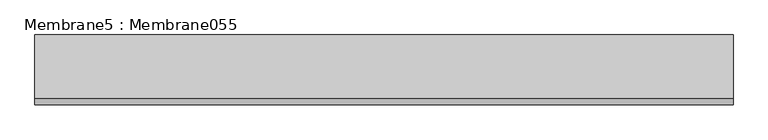
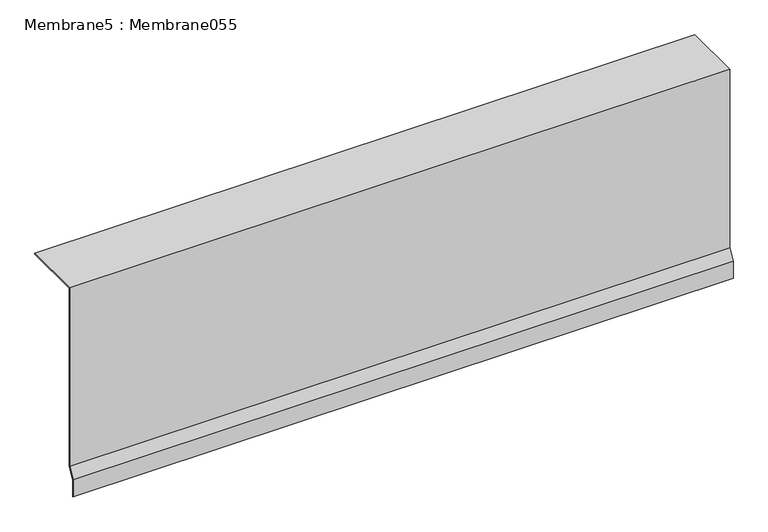
"""IFC4 building model written with IfcOpenShell, lengths in millimetres: proxy geometry, Membrane5 : Membrane055."""

import ifcopenshell
import ifcopenshell.guid

model = None  # the IFC model being written
_history = None  # IfcOwnerHistory: only IFC2X3 demands one
_inside = {}  # id of a spatial element -> (the spatial element, [elements in it])
_under = {}  # id of a project, library or spatial element -> (it, [spatial elements below it])
_declared = {}  # id of a project -> (the project, [libraries it declares])
_typed = {}  # id of a type object -> (the type object, [elements of that type])
_made_of = {}  # id of a material, layer set ... -> (it, [elements and type objects made of it])


def new_model(schema):
    """Start an empty IFC model of exactly this schema.

    Asked for "IFC4X3", IfcOpenShell would pick the latest addendum, in which some entities
    have other attributes; the version numbers below select the first issue.
    IFC2X3 requires an IfcOwnerHistory on every rooted entity: one is made here for all.
    """
    global model, _history
    if schema == "IFC4X3":
        model = ifcopenshell.file(schema_version=(4, 3, 0, 0))
    else:
        model = ifcopenshell.file(schema=schema)
    _inside.clear()
    _under.clear()
    _declared.clear()
    _typed.clear()
    _made_of.clear()
    _history = None
    if model.schema == "IFC2X3":
        org = make("IfcOrganization", Name="unknown")
        user = make(
            "IfcPersonAndOrganization",
            ThePerson=make("IfcPerson", FamilyName="unknown"),
            TheOrganization=org,
        )
        app = make(
            "IfcApplication",
            ApplicationDeveloper=org,
            Version="unknown",
            ApplicationFullName="unknown",
            ApplicationIdentifier="unknown",
        )
        _history = make(
            "IfcOwnerHistory",
            OwningUser=user,
            OwningApplication=app,
            ChangeAction="ADDED",
            CreationDate=0,
        )
    return model


def make(cls, **values):
    """One entity of the class cls with the attributes given. An attribute that is None is left unset."""
    return model.create_entity(
        cls, **{name: value for name, value in values.items() if value is not None}
    )


def rooted(cls, **values):
    """An entity with a GlobalId (a new one), such as an element, a storey or a relation."""
    return make(cls, GlobalId=ifcopenshell.guid.new(), OwnerHistory=_history, **values)


def si_unit(unit_type, name, prefix=None):
    """IfcSIUnit, for example si_unit("LENGTHUNIT", "METRE", prefix="MILLI")."""
    return make("IfcSIUnit", UnitType=unit_type, Prefix=prefix, Name=name)


def assignment(units):
    """IfcUnitAssignment: the units of a project."""
    return None if units is None else make("IfcUnitAssignment", Units=units)


def point(xyz):
    """IfcCartesianPoint."""
    return None if xyz is None else make("IfcCartesianPoint", Coordinates=xyz)


def direction(xyz):
    """IfcDirection."""
    return None if xyz is None else make("IfcDirection", DirectionRatios=xyz)


def frame(location, z_axis=None, x_axis=None):
    """IfcAxis2Placement3D, a coordinate frame: its origin and axes. An axis left out is left unset."""
    return make(
        "IfcAxis2Placement3D",
        Location=point(location),
        Axis=direction(z_axis),
        RefDirection=direction(x_axis),
    )


def origin():
    """The frame at (0, 0, 0) with its axes left unset."""
    return frame((0.0, 0.0, 0.0))


def place(relative_to, where):
    """IfcLocalPlacement: puts the frame where relative to a parent placement (None: the world)."""
    return make(
        "IfcLocalPlacement", PlacementRelTo=relative_to, RelativePlacement=where
    )


def context(
    kind, dimensions, precision=None, world=None, true_north=None, identifier=None
):
    """IfcGeometricRepresentationContext, for example the 3D "Model" context."""
    return make(
        "IfcGeometricRepresentationContext",
        ContextIdentifier=identifier,
        ContextType=kind,
        CoordinateSpaceDimension=dimensions,
        Precision=precision,
        WorldCoordinateSystem=world,
        TrueNorth=true_north,
    )


def project(units=None, contexts=None):
    """IfcProject with its units and contexts."""
    return rooted(
        "IfcProject",
        Name="project",
        RepresentationContexts=contexts,
        UnitsInContext=assignment(units),
    )


def spatial(cls, under=None, at=None, **own):
    """A site, building, storey or space (cls), placed at a placement, below another one or the project."""
    s = rooted(cls, ObjectPlacement=at, **own)
    if under is not None:
        _under.setdefault(under.id(), (under, []))[1].append(s)
    return s


def polyline(points):
    """IfcPolyline through the points."""
    return make("IfcPolyline", Points=[point(p) for p in points])


def outline(outer, holes=None, kind="AREA"):
    """IfcArbitraryClosedProfileDef: a profile drawn as a closed curve; with holes, ...WithVoids."""
    if holes is None:
        return make("IfcArbitraryClosedProfileDef", ProfileType=kind, OuterCurve=outer)
    return make(
        "IfcArbitraryProfileDefWithVoids",
        ProfileType=kind,
        OuterCurve=outer,
        InnerCurves=holes,
    )


def extrude(swept, where, along, depth):
    """IfcExtrudedAreaSolid: the profile swept, set in the frame where, extruded along a direction by depth."""
    return make(
        "IfcExtrudedAreaSolid",
        SweptArea=swept,
        Position=where,
        ExtrudedDirection=direction(along),
        Depth=depth,
    )


def shape(context_of_items, identifier, shape_type, items):
    """IfcShapeRepresentation: the items that make up one representation, for example the "Body"."""
    return make(
        "IfcShapeRepresentation",
        ContextOfItems=context_of_items,
        RepresentationIdentifier=identifier,
        RepresentationType=shape_type,
        Items=items,
    )


def source(mapping_origin, context_of_items, identifier, shape_type, items):
    """IfcRepresentationMap: a shape defined once, which mapped items show again and again."""
    return make(
        "IfcRepresentationMap",
        MappingOrigin=mapping_origin,
        MappedRepresentation=shape(context_of_items, identifier, shape_type, items),
    )


def transform(
    local_origin,
    x_axis=None,
    y_axis=None,
    z_axis=None,
    scale=None,
    scale2=None,
    scale3=None,
    uniform=True,
):
    """IfcCartesianTransformationOperator3D, or its non-uniform kind. x_axis, y_axis, z_axis: its Axis1, 2, 3."""
    if uniform:
        return make(
            "IfcCartesianTransformationOperator3D",
            Axis1=direction(x_axis),
            Axis2=direction(y_axis),
            LocalOrigin=point(local_origin),
            Scale=scale,
            Axis3=direction(z_axis),
        )
    return make(
        "IfcCartesianTransformationOperator3DnonUniform",
        Axis1=direction(x_axis),
        Axis2=direction(y_axis),
        LocalOrigin=point(local_origin),
        Scale=scale,
        Axis3=direction(z_axis),
        Scale2=scale2,
        Scale3=scale3,
    )


def mapped(mapping_source, mapping_target):
    """IfcMappedItem: shows the shape of a source again, moved by a transform."""
    return make(
        "IfcMappedItem", MappingSource=mapping_source, MappingTarget=mapping_target
    )


def made_of(thing, what):
    """Note that an element or type object is made of a material, layer set ...; save() writes the relation."""
    if what is not None:
        _made_of.setdefault(what.id(), (what, []))[1].append(thing)
    return thing


def element(
    cls,
    number,
    at=None,
    inside=None,
    cuts=None,
    type_object=None,
    material=None,
    context=None,
    identifier="Body",
    shape_type=None,
    held_by="IfcProductDefinitionShape",
    body=None,
    shapes=None,
    **own,
):
    """One element of the class cls, such as IfcWall. Its Tag is "e" and its number.

    at: its placement. inside: the storey or other place that contains it. cuts: it is an
    opening in that element (IfcRelVoidsElement). A single representation is given by context,
    identifier, shape_type and body (its items); several are given by shapes. held_by: the class
    of the entity that holds the representations. save() writes the other relations.
    """
    e = rooted(cls, Tag="e%d" % number, ObjectPlacement=at, **own)
    if body is not None:
        shapes = [shape(context, identifier, shape_type, body)]
    if shapes is not None:
        e.Representation = make(held_by, Representations=shapes)
    if inside is not None:
        _inside.setdefault(inside.id(), (inside, []))[1].append(e)
    if cuts is not None:
        rooted(
            "IfcRelVoidsElement", RelatingBuildingElement=cuts, RelatedOpeningElement=e
        )
    if type_object is not None:
        _typed.setdefault(type_object.id(), (type_object, []))[1].append(e)
    return made_of(e, material)


def aggregate(whole, parts):
    """IfcRelAggregates: a whole, such as a stair, and the parts it consists of."""
    return rooted("IfcRelAggregates", RelatingObject=whole, RelatedObjects=parts)


def save(model, path):
    """Write the relations noted so far, then the file.

    IfcRelAggregates (storeys below a building ...), IfcRelContainedInSpatialStructure (elements
    in a storey), IfcRelDefinesByType, IfcRelAssociatesMaterial and IfcRelDeclares: one each for
    every whole, place, type object, material and project.
    """
    for whole, parts in _under.values():
        aggregate(whole, parts)
    for where, things in _inside.values():
        rooted(
            "IfcRelContainedInSpatialStructure",
            RelatedElements=things,
            RelatingStructure=where,
        )
    for kind, things in _typed.values():
        rooted("IfcRelDefinesByType", RelatedObjects=things, RelatingType=kind)
    for what, things in _made_of.values():
        rooted("IfcRelAssociatesMaterial", RelatedObjects=things, RelatingMaterial=what)
    for by, libraries in _declared.values():
        rooted("IfcRelDeclares", RelatingContext=by, RelatedDefinitions=libraries)
    model.write(path)


def membrane5_membrane055_e15eec0d(model_context):
    return source(origin(), model_context, "Body", "SweptSolid", [
        extrude(outline(polyline([(-5540.3481445, 40225.0071475), (-5358.6630859, 40225.0071475), (-5358.6630859, 40223.0071475), (-5538.3481445, 40223.0071475), (-5538.3481445, 39652.5453283), (-5556.9582483, 39620.311683), (-5556.9582483, 39566.6060938), (-5558.9582483, 39566.6060938), (-5558.9582483, 39620.8475814), (-5540.3481445, 39653.0812267), (-5540.3481445, 40225.0071475)])), frame((12383.1678845, 0.0, 0.0), z_axis=(1.0, 0.0, 0.0), x_axis=(0.0, 1.0, 0.0)), (0.0, 0.0, 1.0), 1999.85),
    ])


if __name__ == "__main__":
    model = new_model("IFC4")
    model_context = context("Model", 3, world=origin())
    ifc_project = project(units=[si_unit("LENGTHUNIT", "METRE", prefix="MILLI")], contexts=[model_context])
    site = spatial("IfcSite", under=ifc_project)
    building = spatial("IfcBuilding", under=site)
    placement = place(None, origin())
    membrane5_membrane055_shape = membrane5_membrane055_e15eec0d(model_context)
    element("IfcBuildingElementProxy", 1, Name="Membrane5 : Membrane055", ObjectType="Membrane5 : Membrane055", at=placement, inside=building, context=model_context, shape_type="MappedRepresentation", body=[
        mapped(membrane5_membrane055_shape, transform((0.0, 0.0, 0.0), x_axis=(1.0, 0.0, 0.0), y_axis=(0.0, 1.0, 0.0), z_axis=(0.0, 0.0, 1.0))),
    ])
    save(model, "model.ifc")

# Revit data of these elements
# Type "Membrane5 : Membrane055"
#   NameOverride = "Membrane055"
# Element 1 (IfcBuildingElementProxy, "Membrane5 : Membrane055")
#   Materials on its faces: "(2) LAYERS OF ICE & WATER SHIELD (BITUTHANE) UNDER STUCCO"
# Materials
#   "(2) LAYERS OF ICE & WATER SHIELD (BITUTHANE) UNDER STUCCO": class "Unassigned", colour RGB 186 255 159, transparency 0, Cost = 0
